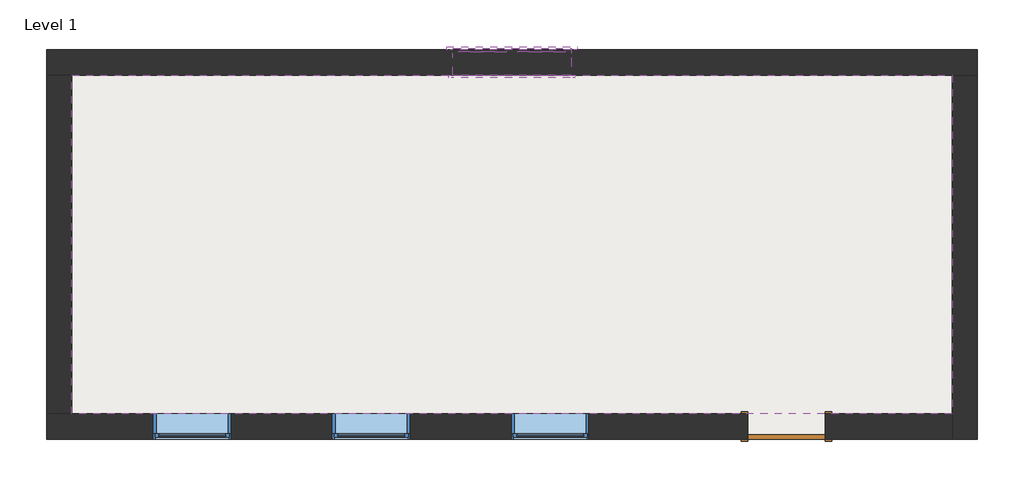
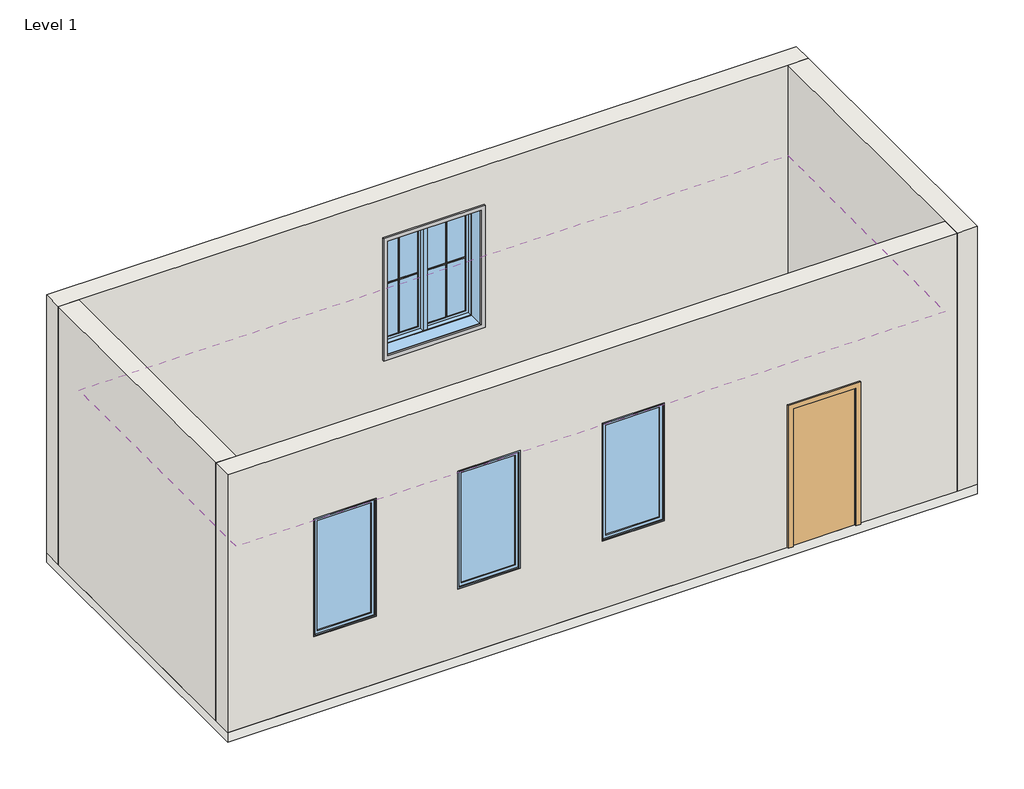
# One storey: 4 proxies, 4 walls, 4 windows, 1 covering, 1 door, 1 slab.
"""IFC4 building model written with IfcOpenShell, lengths in millimetres."""

import ifcopenshell
import ifcopenshell.guid

model = None  # the IFC model being written
_history = None  # IfcOwnerHistory: only IFC2X3 demands one
_inside = {}  # id of a spatial element -> (the spatial element, [elements in it])
_under = {}  # id of a project, library or spatial element -> (it, [spatial elements below it])
_declared = {}  # id of a project -> (the project, [libraries it declares])
_typed = {}  # id of a type object -> (the type object, [elements of that type])
_made_of = {}  # id of a material, layer set ... -> (it, [elements and type objects made of it])


def new_model(schema):
    """Start an empty IFC model of exactly this schema.

    Asked for "IFC4X3", IfcOpenShell would pick the latest addendum, in which some entities
    have other attributes; the version numbers below select the first issue.
    IFC2X3 requires an IfcOwnerHistory on every rooted entity: one is made here for all.
    """
    global model, _history
    if schema == "IFC4X3":
        model = ifcopenshell.file(schema_version=(4, 3, 0, 0))
    else:
        model = ifcopenshell.file(schema=schema)
    _inside.clear()
    _under.clear()
    _declared.clear()
    _typed.clear()
    _made_of.clear()
    _history = None
    if model.schema == "IFC2X3":
        org = make("IfcOrganization", Name="unknown")
        user = make(
            "IfcPersonAndOrganization",
            ThePerson=make("IfcPerson", FamilyName="unknown"),
            TheOrganization=org,
        )
        app = make(
            "IfcApplication",
            ApplicationDeveloper=org,
            Version="unknown",
            ApplicationFullName="unknown",
            ApplicationIdentifier="unknown",
        )
        _history = make(
            "IfcOwnerHistory",
            OwningUser=user,
            OwningApplication=app,
            ChangeAction="ADDED",
            CreationDate=0,
        )
    return model


def make(cls, **values):
    """One entity of the class cls with the attributes given. An attribute that is None is left unset."""
    return model.create_entity(
        cls, **{name: value for name, value in values.items() if value is not None}
    )


def rooted(cls, **values):
    """An entity with a GlobalId (a new one), such as an element, a storey or a relation."""
    return make(cls, GlobalId=ifcopenshell.guid.new(), OwnerHistory=_history, **values)


def si_unit(unit_type, name, prefix=None):
    """IfcSIUnit, for example si_unit("LENGTHUNIT", "METRE", prefix="MILLI")."""
    return make("IfcSIUnit", UnitType=unit_type, Prefix=prefix, Name=name)


def assignment(units):
    """IfcUnitAssignment: the units of a project."""
    return None if units is None else make("IfcUnitAssignment", Units=units)


def point(xyz):
    """IfcCartesianPoint."""
    return None if xyz is None else make("IfcCartesianPoint", Coordinates=xyz)


def direction(xyz):
    """IfcDirection."""
    return None if xyz is None else make("IfcDirection", DirectionRatios=xyz)


def frame(location, z_axis=None, x_axis=None):
    """IfcAxis2Placement3D, a coordinate frame: its origin and axes. An axis left out is left unset."""
    return make(
        "IfcAxis2Placement3D",
        Location=point(location),
        Axis=direction(z_axis),
        RefDirection=direction(x_axis),
    )


def origin():
    """The frame at (0, 0, 0) with its axes left unset."""
    return frame((0.0, 0.0, 0.0))


def origin_with_axes():
    """The frame at (0, 0, 0) with the z axis (0, 0, 1) and the x axis (1, 0, 0) written out."""
    return frame((0.0, 0.0, 0.0), z_axis=(0.0, 0.0, 1.0), x_axis=(1.0, 0.0, 0.0))


def place(relative_to, where):
    """IfcLocalPlacement: puts the frame where relative to a parent placement (None: the world)."""
    return make(
        "IfcLocalPlacement", PlacementRelTo=relative_to, RelativePlacement=where
    )


def context(
    kind, dimensions, precision=None, world=None, true_north=None, identifier=None
):
    """IfcGeometricRepresentationContext, for example the 3D "Model" context."""
    return make(
        "IfcGeometricRepresentationContext",
        ContextIdentifier=identifier,
        ContextType=kind,
        CoordinateSpaceDimension=dimensions,
        Precision=precision,
        WorldCoordinateSystem=world,
        TrueNorth=true_north,
    )


def project(units=None, contexts=None):
    """IfcProject with its units and contexts."""
    return rooted(
        "IfcProject",
        Name="project",
        RepresentationContexts=contexts,
        UnitsInContext=assignment(units),
    )


def spatial(cls, under=None, at=None, **own):
    """A site, building, storey or space (cls), placed at a placement, below another one or the project."""
    s = rooted(cls, ObjectPlacement=at, **own)
    if under is not None:
        _under.setdefault(under.id(), (under, []))[1].append(s)
    return s


def polyline(points):
    """IfcPolyline through the points."""
    return make("IfcPolyline", Points=[point(p) for p in points])


def outline(outer, holes=None, kind="AREA"):
    """IfcArbitraryClosedProfileDef: a profile drawn as a closed curve; with holes, ...WithVoids."""
    if holes is None:
        return make("IfcArbitraryClosedProfileDef", ProfileType=kind, OuterCurve=outer)
    return make(
        "IfcArbitraryProfileDefWithVoids",
        ProfileType=kind,
        OuterCurve=outer,
        InnerCurves=holes,
    )


def extrude(swept, where, along, depth):
    """IfcExtrudedAreaSolid: the profile swept, set in the frame where, extruded along a direction by depth."""
    return make(
        "IfcExtrudedAreaSolid",
        SweptArea=swept,
        Position=where,
        ExtrudedDirection=direction(along),
        Depth=depth,
    )


def faces_of(points, faces, orient=None, outer=None):
    """IfcFace entities. A face is a list of loops; a loop is a list of indices into points, from 0.

    orient and outer hold one flag for each loop. By default every Orientation is true, the
    first loop of a face is its IfcFaceOuterBound and the others are IfcFaceBound.
    """
    made = []
    for i, loops in enumerate(faces):
        bounds = []
        for j, loop in enumerate(loops):
            is_outer = j == 0 if outer is None else outer[i][j]
            bounds.append(
                make(
                    "IfcFaceOuterBound" if is_outer else "IfcFaceBound",
                    Bound=make("IfcPolyLoop", Polygon=[points[k] for k in loop]),
                    Orientation=True if orient is None else orient[i][j],
                )
            )
        made.append(make("IfcFace", Bounds=bounds))
    return made


def faceted_brep(points, faces, orient=None, outer=None, voids=None):
    """IfcFacetedBrep: a solid bounded by flat faces; with voids (closed shells), ...WithVoids."""
    shared = [point(p) for p in points]
    hull = make("IfcClosedShell", CfsFaces=faces_of(shared, faces, orient, outer))
    if voids is None:
        return make("IfcFacetedBrep", Outer=hull)
    return make(
        "IfcFacetedBrepWithVoids",
        Outer=hull,
        Voids=[
            make(cls, CfsFaces=faces_of(shared, fs, o, b)) for cls, fs, o, b in voids
        ],
    )


def shape(context_of_items, identifier, shape_type, items):
    """IfcShapeRepresentation: the items that make up one representation, for example the "Body"."""
    return make(
        "IfcShapeRepresentation",
        ContextOfItems=context_of_items,
        RepresentationIdentifier=identifier,
        RepresentationType=shape_type,
        Items=items,
    )


def source(mapping_origin, context_of_items, identifier, shape_type, items):
    """IfcRepresentationMap: a shape defined once, which mapped items show again and again."""
    return make(
        "IfcRepresentationMap",
        MappingOrigin=mapping_origin,
        MappedRepresentation=shape(context_of_items, identifier, shape_type, items),
    )


def transform(
    local_origin,
    x_axis=None,
    y_axis=None,
    z_axis=None,
    scale=None,
    scale2=None,
    scale3=None,
    uniform=True,
):
    """IfcCartesianTransformationOperator3D, or its non-uniform kind. x_axis, y_axis, z_axis: its Axis1, 2, 3."""
    if uniform:
        return make(
            "IfcCartesianTransformationOperator3D",
            Axis1=direction(x_axis),
            Axis2=direction(y_axis),
            LocalOrigin=point(local_origin),
            Scale=scale,
            Axis3=direction(z_axis),
        )
    return make(
        "IfcCartesianTransformationOperator3DnonUniform",
        Axis1=direction(x_axis),
        Axis2=direction(y_axis),
        LocalOrigin=point(local_origin),
        Scale=scale,
        Axis3=direction(z_axis),
        Scale2=scale2,
        Scale3=scale3,
    )


def mapped(mapping_source, mapping_target):
    """IfcMappedItem: shows the shape of a source again, moved by a transform."""
    return make(
        "IfcMappedItem", MappingSource=mapping_source, MappingTarget=mapping_target
    )


def made_of(thing, what):
    """Note that an element or type object is made of a material, layer set ...; save() writes the relation."""
    if what is not None:
        _made_of.setdefault(what.id(), (what, []))[1].append(thing)
    return thing


def element(
    cls,
    number,
    at=None,
    inside=None,
    cuts=None,
    type_object=None,
    material=None,
    context=None,
    identifier="Body",
    shape_type=None,
    held_by="IfcProductDefinitionShape",
    body=None,
    shapes=None,
    **own,
):
    """One element of the class cls, such as IfcWall. Its Tag is "e" and its number.

    at: its placement. inside: the storey or other place that contains it. cuts: it is an
    opening in that element (IfcRelVoidsElement). A single representation is given by context,
    identifier, shape_type and body (its items); several are given by shapes. held_by: the class
    of the entity that holds the representations. save() writes the other relations.
    """
    e = rooted(cls, Tag="e%d" % number, ObjectPlacement=at, **own)
    if body is not None:
        shapes = [shape(context, identifier, shape_type, body)]
    if shapes is not None:
        e.Representation = make(held_by, Representations=shapes)
    if inside is not None:
        _inside.setdefault(inside.id(), (inside, []))[1].append(e)
    if cuts is not None:
        rooted(
            "IfcRelVoidsElement", RelatingBuildingElement=cuts, RelatedOpeningElement=e
        )
    if type_object is not None:
        _typed.setdefault(type_object.id(), (type_object, []))[1].append(e)
    return made_of(e, material)


def aggregate(whole, parts):
    """IfcRelAggregates: a whole, such as a stair, and the parts it consists of."""
    return rooted("IfcRelAggregates", RelatingObject=whole, RelatedObjects=parts)


def save(model, path):
    """Write the relations noted so far, then the file.

    IfcRelAggregates (storeys below a building ...), IfcRelContainedInSpatialStructure (elements
    in a storey), IfcRelDefinesByType, IfcRelAssociatesMaterial and IfcRelDeclares: one each for
    every whole, place, type object, material and project.
    """
    for whole, parts in _under.values():
        aggregate(whole, parts)
    for where, things in _inside.values():
        rooted(
            "IfcRelContainedInSpatialStructure",
            RelatedElements=things,
            RelatingStructure=where,
        )
    for kind, things in _typed.values():
        rooted("IfcRelDefinesByType", RelatedObjects=things, RelatingType=kind)
    for what, things in _made_of.values():
        rooted("IfcRelAssociatesMaterial", RelatedObjects=things, RelatingMaterial=what)
    for by, libraries in _declared.values():
        rooted("IfcRelDeclares", RelatingContext=by, RelatedDefinitions=libraries)
    model.write(path)


def m_muntin_pattern_2x2_m_muntin_pattern_2x2_d2d4b859(model_context):
    return source(origin(), model_context, "Body", "SweptSolid", [
        extrude(outline(polyline([(836.5, -6.35), (836.5, -281.7375), (823.8, -281.7375), (823.8, -6.35), (0.0, -6.35), (0.0, 6.35), (823.8, 6.35), (823.8, 281.7375), (836.5, 281.7375), (836.5, 6.35), (1660.3, 6.35), (1660.3, -6.35), (836.5, -6.35)])), frame((0.0, 9.525, 0.0), z_axis=(0.0, 1.0, 0.0), x_axis=(0.0, 0.0, 1.0)), (0.0, 0.0, 1.0), 12.7),
        extrude(outline(polyline([(836.5, -6.35), (836.5, -281.7375), (823.8, -281.7375), (823.8, -6.35), (0.0, -6.35), (0.0, 6.35), (823.8, 6.35), (823.8, 281.7375), (836.5, 281.7375), (836.5, 6.35), (1660.3, 6.35), (1660.3, -6.35), (836.5, -6.35)])), frame((0.0, -22.225, 0.0), z_axis=(0.0, 1.0, 0.0), x_axis=(0.0, 0.0, 1.0)), (0.0, 0.0, 1.0), 12.7),
    ])


def m_muntin_pattern_2x2_m_muntin_pattern_2x2_f3921bb5(model_context):
    return source(origin(), model_context, "Body", "SweptSolid", [
        extrude(outline(polyline([(836.5, -6.35), (836.5, -281.7375), (823.8, -281.7375), (823.8, -6.35), (0.0, -6.35), (0.0, 6.35), (823.8, 6.35), (823.8, 281.7375), (836.5, 281.7375), (836.5, 6.35), (1660.3, 6.35), (1660.3, -6.35), (836.5, -6.35)])), frame((0.0, -22.225, 0.0), z_axis=(0.0, 1.0, 0.0), x_axis=(0.0, 0.0, 1.0)), (0.0, 0.0, 1.0), 12.7),
        extrude(outline(polyline([(836.5, -6.35), (836.5, -281.7375), (823.8, -281.7375), (823.8, -6.35), (0.0, -6.35), (0.0, 6.35), (823.8, 6.35), (823.8, 281.7375), (836.5, 281.7375), (836.5, 6.35), (1660.3, 6.35), (1660.3, -6.35), (836.5, -6.35)])), frame((0.0, 9.525, 0.0), z_axis=(0.0, 1.0, 0.0), x_axis=(0.0, 0.0, 1.0)), (0.0, 0.0, 1.0), 12.7),
    ])


def m_trim_window_exterior_flat_with_sill_136e302d(model_context):
    return source(origin(), model_context, "Body", "SweptSolid", [
        extrude(outline(polyline([(760.0, -1820.4323709), (760.0, -1880.4323709), (-760.0, -1880.4323709), (-760.0, -1820.4323709), (760.0, -1820.4323709)])), origin_with_axes(), (0.0, 0.0, 1.0), 19.05),
        extrude(outline(polyline([(-1830.0, 38.1), (-1802.4580645, 38.1), (-1800.0, 19.05), (-1800.0, 0.0), (-1820.4323709, 0.0), (-1820.4323709, 19.05), (-1830.0, 19.05), (-1830.0, 38.1)])), frame((-772.7, 0.0, 0.0), z_axis=(1.0, 0.0, 0.0), x_axis=(0.0, 1.0, 0.0)), (0.0, 0.0, 1.0), 1545.4),
        extrude(outline(polyline([(-760.0, 60.0), (760.0, 60.0), (760.0, -1800.0), (700.0, -1800.0), (700.0, 0.0), (-700.0, 0.0), (-700.0, -1800.0), (-760.0, -1800.0), (-760.0, 60.0)])), origin_with_axes(), (0.0, 0.0, 1.0), 19.05),
    ])


def m_trim_window_interior_flat_picture_frame_c6c50358(model_context):
    return source(origin(), model_context, "Body", "SweptSolid", [
        extrude(outline(polyline([(747.3, 47.3), (747.3, -1847.3), (-747.3, -1847.3), (-747.3, 47.3), (747.3, 47.3)]), holes=[polyline([(687.3, -12.7), (-687.3, -12.7), (-687.3, -1787.3), (687.3, -1787.3), (687.3, -12.7)])]), origin_with_axes(), (0.0, 0.0, 1.0), 30.0),
    ])


def m_single_flush_0915_x_2134mm_9cebaac8(model_context):
    return source(origin(), model_context, "Body", "SweptSolid", [
        extrude(outline(polyline([(2210.0, -533.5), (0.0, -533.5), (0.0, -457.5), (2134.0, -457.5), (2134.0, 457.5), (0.0, 457.5), (0.0, 533.5), (2210.0, 533.5), (2210.0, -533.5)])), frame((0.0, 150.0, 0.0), z_axis=(0.0, 1.0, 0.0), x_axis=(0.0, 0.0, 1.0)), (0.0, 0.0, 1.0), 25.0),
        extrude(outline(polyline([(2210.0, 533.5), (2210.0, -533.5), (0.0, -533.5), (0.0, -457.5), (2134.0, -457.5), (2134.0, 457.5), (0.0, 457.5), (0.0, 533.5), (2210.0, 533.5)])), frame((0.0, -175.0, 0.0), z_axis=(0.0, 1.0, 0.0), x_axis=(0.0, 0.0, 1.0)), (0.0, 0.0, 1.0), 25.0),
        extrude(outline(polyline([(457.5, 99.0), (-457.5, 99.0), (-457.5, 150.0), (457.5, 150.0), (457.5, 99.0)])), origin_with_axes(), (0.0, 0.0, 1.0), 2134.0),
    ])


def m_fixed_0915_x_1830mm_2a137b51(model_context):
    return source(origin(), model_context, "Body", "SweptSolid", [
        extrude(outline(polyline([(-394.5, 128.0), (394.5, 128.0), (394.5, 116.0), (-394.5, 116.0), (-394.5, 128.0)])), frame((0.0, 0.0, 368.0), z_axis=(0.0, 0.0, 1.0), x_axis=(1.0, 0.0, 0.0)), (0.0, 0.0, 1.0), 1704.0),
        extrude(outline(polyline([(2116.0, -438.5), (324.0, -438.5), (324.0, 438.5), (2116.0, 438.5), (2116.0, -438.5)]), holes=[polyline([(2072.0, -394.5), (2072.0, 394.5), (368.0, 394.5), (368.0, -394.5), (2072.0, -394.5)])]), frame((0.0, 100.0, 0.0), z_axis=(0.0, 1.0, 0.0), x_axis=(0.0, 0.0, 1.0)), (0.0, 0.0, 1.0), 44.0),
        extrude(outline(polyline([(2135.0, -457.5), (305.0, -457.5), (305.0, 457.5), (2135.0, 457.5), (2135.0, -457.5)]), holes=[polyline([(2116.0, -438.5), (2116.0, 438.5), (324.0, 438.5), (324.0, -438.5), (2116.0, -438.5)])]), frame((0.0, 100.0, 0.0), z_axis=(0.0, 1.0, 0.0), x_axis=(0.0, 0.0, 1.0)), (0.0, 0.0, 1.0), 63.0),
        extrude(outline(polyline([(2135.0, -457.5), (305.0, -457.5), (305.0, 457.5), (2135.0, 457.5), (2135.0, -457.5)]), holes=[polyline([(2103.0, -425.5), (2103.0, 425.5), (337.0, 425.5), (337.0, -425.5), (2103.0, -425.5)])]), frame((0.0, -137.0, 0.0), z_axis=(0.0, 1.0, 0.0), x_axis=(0.0, 0.0, 1.0)), (0.0, 0.0, 1.0), 237.0),
    ])


def m_window_casement_double_1400_x_1800mm_f8d7c7c6(model_context):
    return source(origin(), model_context, "Body", "SolidModel", [
        faceted_brep([(9.525, 169.05, 2687.3), (-9.525, 169.05, 2687.3), (-9.525, 118.25, 2687.3), (9.525, 118.25, 2687.3), (9.525, 169.05, 912.7), (9.525, 118.25, 912.7), (-9.525, 118.25, 912.7), (-9.525, 169.05, 912.7), (-9.525, 118.25, 931.75), (-9.525, 118.25, 2668.25), (-30.1625, 118.25, 931.75), (-30.1625, 118.25, 2668.25), (-30.1625, 54.75, 931.75), (-30.1625, 54.75, 2668.25), (30.1625, 54.75, 931.75), (30.1625, 54.75, 2668.25), (30.1625, 118.25, 931.75), (30.1625, 118.25, 2668.25), (9.525, 118.25, 931.75), (9.525, 118.25, 2668.25)], [[[0, 1, 2, 3]], [[4, 5, 6, 7]], [[1, 0, 4, 7]], [[2, 1, 7, 6, 8, 9]], [[9, 8, 10, 11]], [[11, 10, 12, 13]], [[13, 12, 14, 15]], [[15, 14, 16, 17]], [[17, 16, 18, 19]], [[0, 3, 19, 18, 5, 4]], [[18, 8, 6, 5]], [[9, 19, 3, 2]], [[8, 18, 16, 14, 12, 10]], [[19, 9, 11, 13, 15, 17]]]),
        extrude(outline(polyline([(-66.675, 150.0), (-66.675, 143.65), (-630.15, 143.65), (-630.15, 150.0), (-66.675, 150.0)])), frame((0.0, 0.0, 969.85), z_axis=(0.0, 0.0, 1.0), x_axis=(1.0, 0.0, 0.0)), (0.0, 0.0, 1.0), 1660.3),
        extrude(outline(polyline([(-630.15, 130.95), (-630.15, 137.3), (-66.675, 137.3), (-66.675, 130.95), (-630.15, 130.95)])), frame((0.0, 0.0, 969.85), z_axis=(0.0, 0.0, 1.0), x_axis=(1.0, 0.0, 0.0)), (0.0, 0.0, 1.0), 1660.3),
        extrude(outline(polyline([(630.15, 150.0), (630.15, 143.65), (66.675, 143.65), (66.675, 150.0), (630.15, 150.0)])), frame((0.0, 0.0, 969.85), z_axis=(0.0, 0.0, 1.0), x_axis=(1.0, 0.0, 0.0)), (0.0, 0.0, 1.0), 1660.3),
        extrude(outline(polyline([(66.675, 130.95), (66.675, 137.3), (630.15, 137.3), (630.15, 130.95), (66.675, 130.95)])), frame((0.0, 0.0, 969.85), z_axis=(0.0, 0.0, 1.0), x_axis=(1.0, 0.0, 0.0)), (0.0, 0.0, 1.0), 1660.3),
        extrude(outline(polyline([(2687.3, -687.3), (912.7, -687.3), (912.7, -9.525), (2687.3, -9.525), (2687.3, -687.3)]), holes=[polyline([(2630.15, -66.675), (969.85, -66.675), (969.85, -630.15), (2630.15, -630.15), (2630.15, -66.675)])]), frame((0.0, 118.25, 0.0), z_axis=(0.0, 1.0, 0.0), x_axis=(0.0, 0.0, 1.0)), (0.0, 0.0, 1.0), 44.45),
        extrude(outline(polyline([(912.7, 687.3), (2687.3, 687.3), (2687.3, 9.525), (912.7, 9.525), (912.7, 687.3)]), holes=[polyline([(969.85, 66.675), (2630.15, 66.675), (2630.15, 630.15), (969.85, 630.15), (969.85, 66.675)])]), frame((0.0, 118.25, 0.0), z_axis=(0.0, 1.0, 0.0), x_axis=(0.0, 0.0, 1.0)), (0.0, 0.0, 1.0), 44.45),
        extrude(outline(polyline([(2700.0, -700.0), (900.0, -700.0), (900.0, 700.0), (2700.0, 700.0), (2700.0, -700.0)]), holes=[polyline([(2680.95, 680.95), (919.05, 680.95), (919.05, -680.95), (2680.95, -680.95), (2680.95, 680.95)])]), frame((0.0, -150.0, 0.0), z_axis=(0.0, 1.0, 0.0), x_axis=(0.0, 0.0, 1.0)), (0.0, 0.0, 1.0), 204.75),
        faceted_brep([(668.25, 118.25, 2668.25), (668.25, 54.75, 2668.25), (-668.25, 54.75, 2668.25), (-668.25, 118.25, 2668.25), (687.3, 169.05, 2687.3), (687.3, 118.25, 2687.3), (-687.3, 118.25, 2687.3), (-687.3, 169.05, 2687.3), (700.0, 54.75, 2700.0), (700.0, 169.05, 2700.0), (-700.0, 169.05, 2700.0), (-700.0, 54.75, 2700.0), (-668.25, 54.75, 931.75), (-668.25, 118.25, 931.75), (-687.3, 118.25, 912.7), (-687.3, 169.05, 912.7), (-700.0, 169.05, 900.0), (-700.0, 54.75, 900.0), (668.25, 54.75, 931.75), (668.25, 118.25, 931.75), (687.3, 118.25, 912.7), (687.3, 169.05, 912.7), (700.0, 169.05, 900.0), (700.0, 54.75, 900.0)], [[[0, 1, 2, 3]], [[4, 5, 6, 7]], [[8, 9, 10, 11]], [[3, 2, 12, 13]], [[7, 6, 14, 15]], [[11, 10, 16, 17]], [[13, 12, 18, 19]], [[15, 14, 20, 21]], [[17, 16, 22, 23]], [[11, 17, 23, 8], [1, 18, 12, 2]], [[19, 18, 1, 0]], [[5, 20, 14, 6], [3, 13, 19, 0]], [[21, 20, 5, 4]], [[23, 22, 9, 8]], [[9, 22, 16, 10], [7, 15, 21, 4]]]),
    ])


model = new_model("IFC4")

# Units and contexts
model_context = context("Model", 3, world=origin())
ifc_project = project(units=[si_unit("LENGTHUNIT", "METRE", prefix="MILLI")], contexts=[model_context])

# Site, building, storey
site = spatial("IfcSite", under=ifc_project)
building = spatial("IfcBuilding", under=site)
storey = spatial("IfcBuildingStorey", under=building, Name="Level 1", Elevation=0.0)

# Proxies
placement = place(None, origin())
m_muntin_pattern_2x2_m_muntin_pattern_2x2_shape = m_muntin_pattern_2x2_m_muntin_pattern_2x2_d2d4b859(model_context)
element("IfcBuildingElementProxy", 1, Name="M_Muntin Pattern_2x2 : M_Muntin Pattern_2x2", ObjectType="M_Muntin Pattern_2x2 : M_Muntin Pattern_2x2", at=placement, inside=storey, context=model_context, shape_type="MappedRepresentation", body=[
    mapped(m_muntin_pattern_2x2_m_muntin_pattern_2x2_shape, transform((3955.3182322, 4425.5280909, 1625.687058), x_axis=(1.0, 0.0, 0.0), y_axis=(0.0, 1.0, 0.0), z_axis=(0.0, 0.0, 1.0))),
])
m_muntin_pattern_2x2_m_muntin_pattern_2x2_2_shape = m_muntin_pattern_2x2_m_muntin_pattern_2x2_f3921bb5(model_context)
element("IfcBuildingElementProxy", 2, Name="M_Muntin Pattern_2x2 : M_Muntin Pattern_2x2", ObjectType="M_Muntin Pattern_2x2 : M_Muntin Pattern_2x2", at=placement, inside=storey, context=model_context, shape_type="MappedRepresentation", body=[
    mapped(m_muntin_pattern_2x2_m_muntin_pattern_2x2_2_shape, transform((4652.1432322, 4425.5280909, 1625.687058), x_axis=(-1.0, 0.0, 0.0), y_axis=(0.0, -1.0, 0.0), z_axis=(0.0, 0.0, 1.0))),
])
m_trim_window_exterior_flat_with_sill_shape = m_trim_window_exterior_flat_with_sill_136e302d(model_context)
element("IfcBuildingElementProxy", 3, Name="M_Trim-Window-Exterior-Flat : with Sill", ObjectType="M_Trim-Window-Exterior-Flat : with Sill", at=placement, inside=storey, context=model_context, shape_type="MappedRepresentation", body=[
    mapped(m_trim_window_exterior_flat_with_sill_shape, transform((4303.7307322, 4435.0530909, 3355.837058), x_axis=(-1.0, 0.0, 0.0), y_axis=(0.0, 0.0, 1.0), z_axis=(0.0, 1.0, 0.0))),
])
m_trim_window_interior_flat_picture_frame_shape = m_trim_window_interior_flat_picture_frame_c6c50358(model_context)
element("IfcBuildingElementProxy", 4, Name="M_Trim-Window-Interior-Flat : Picture Frame", ObjectType="M_Trim-Window-Interior-Flat : Picture Frame", at=placement, inside=storey, context=model_context, shape_type="MappedRepresentation", body=[
    mapped(m_trim_window_interior_flat_picture_frame_shape, transform((4303.7307322, 4135.0530909, 3355.837058), x_axis=(1.0, 0.0, 0.0), y_axis=(0.0, 0.0, 1.0), z_axis=(0.0, -1.0, 0.0))),
])

# Covering
element("IfcCovering", 5, ObjectType="Plain", at=placement, inside=storey, context=model_context, shape_type="SweptSolid", body=[
    extrude(outline(polyline([(-896.2692678, 4135.0530909), (9503.7307322, 4135.0530909), (9503.7307322, 135.0530909), (-896.2692678, 135.0530909), (-896.2692678, 4135.0530909)])), frame((0.0, 0.0, 2600.0), z_axis=(0.0, 0.0, 1.0), x_axis=(1.0, 0.0, 0.0)), (0.0, 0.0, 1.0), 57.0),
])

# Door
m_single_flush_0915_x_2134mm_shape = m_single_flush_0915_x_2134mm_9cebaac8(model_context)
element("IfcDoor", 6, ObjectType="M_Single-Flush : 0915 x 2134mm", at=placement, inside=storey, context=model_context, shape_type="MappedRepresentation", body=[
    mapped(m_single_flush_0915_x_2134mm_shape, transform((7546.2307322, -14.9469091, 0.0), x_axis=(-1.0, 0.0, 0.0), y_axis=(0.0, -1.0, 0.0), z_axis=(0.0, 0.0, 1.0))),
])

# Slab
element("IfcSlab", 7, ObjectType="Generic 150mm", at=placement, inside=storey, context=model_context, shape_type="SweptSolid", body=[
    extrude(outline(polyline([(9803.7307322, 4435.0530909), (9803.7307322, -164.9469091), (-1196.2692678, -164.9469091), (-1196.2692678, 4435.0530909), (9803.7307322, 4435.0530909)])), frame((0.0, 0.0, -150.0), z_axis=(0.0, 0.0, 1.0), x_axis=(1.0, 0.0, 0.0)), (0.0, 0.0, 1.0), 150.0),
])

# Walls
element("IfcWall", 8, ObjectType="Generic - 300mm", at=placement, inside=storey, context=model_context, shape_type="Brep", body=[
    faceted_brep([(-1196.2692678, 4135.0530909, 0.0), (-896.2692678, 4135.0530909, 0.0), (9503.7307322, 4135.0530909, 0.0), (9803.7307322, 4135.0530909, 0.0), (9803.7307322, 4135.0530909, 4000.0), (9503.7307322, 4135.0530909, 4000.0), (-896.2692678, 4135.0530909, 4000.0), (-1196.2692678, 4135.0530909, 4000.0), (5003.7307322, 4135.0530909, 3355.837058), (5003.7307322, 4135.0530909, 1555.837058), (3603.7307322, 4135.0530909, 1555.837058), (3603.7307322, 4135.0530909, 3355.837058), (-1196.2692678, 4435.0530909, 0.0), (-1196.2692678, 4435.0530909, 4000.0), (9803.7307322, 4435.0530909, 4000.0), (9803.7307322, 4435.0530909, 0.0), (5003.7307322, 4435.0530909, 3355.837058), (3603.7307322, 4435.0530909, 3355.837058), (3603.7307322, 4435.0530909, 1555.837058), (5003.7307322, 4435.0530909, 1555.837058)], [[[0, 1, 2, 3, 4, 5, 6, 7], [8, 9, 10, 11]], [[12, 13, 14, 15], [16, 17, 18, 19]], [[3, 2, 1, 0, 12, 15]], [[7, 6, 5, 4, 14, 13]], [[4, 3, 15, 14]], [[0, 7, 13, 12]], [[9, 8, 16, 19]], [[10, 9, 19, 18]], [[11, 10, 18, 17]], [[8, 11, 17, 16]]]),
])
element("IfcWall", 9, ObjectType="Generic - 300mm", at=placement, inside=storey, context=model_context, shape_type="Brep", body=[
    faceted_brep([(9503.7307322, 4135.0530909, 0.0), (9503.7307322, 135.0530909, 0.0), (9503.7307322, -164.9469091, 0.0), (9503.7307322, -164.9469091, 4000.0), (9503.7307322, 135.0530909, 4000.0), (9503.7307322, 4135.0530909, 4000.0), (9803.7307322, 4135.0530909, 0.0), (9803.7307322, 4135.0530909, 4000.0), (9803.7307322, -164.9469091, 4000.0), (9803.7307322, -164.9469091, 0.0)], [[[0, 1, 2, 3, 4, 5]], [[6, 7, 8, 9]], [[2, 1, 0, 6, 9]], [[5, 4, 3, 8, 7]], [[0, 5, 7, 6]], [[3, 2, 9, 8]]]),
])
element("IfcWall", 10, ObjectType="Generic - 300mm", at=placement, inside=storey, context=model_context, shape_type="Brep", body=[
    faceted_brep([(7088.7307322, 135.0530909, 2134.0), (7088.7307322, 135.0530909, 0.0), (-896.2692678, 135.0530909, 0.0), (-1196.2692678, 135.0530909, 0.0), (-1196.2692678, 135.0530909, 4000.0), (-896.2692678, 135.0530909, 4000.0), (9503.7307322, 135.0530909, 4000.0), (9503.7307322, 135.0530909, 0.0), (8003.7307322, 135.0530909, 0.0), (8003.7307322, 135.0530909, 2134.0), (5212.0305123, 135.0530909, 1044.7986801), (5212.0305123, 135.0530909, 2874.7986801), (4297.0305123, 135.0530909, 2874.7986801), (4297.0305123, 135.0530909, 1044.7986801), (3097.0305123, 135.0530909, 1044.7986801), (3097.0305123, 135.0530909, 2874.7986801), (2182.0305123, 135.0530909, 2874.7986801), (2182.0305123, 135.0530909, 1044.7986801), (982.0305123, 135.0530909, 1044.7986801), (982.0305123, 135.0530909, 2874.7986801), (67.0305123, 135.0530909, 2874.7986801), (67.0305123, 135.0530909, 1044.7986801), (-1196.2692678, -164.9469091, 0.0), (7088.7307322, -164.9469091, 0.0), (7088.7307322, -164.9469091, 2134.0), (8003.7307322, -164.9469091, 2134.0), (8003.7307322, -164.9469091, 0.0), (9503.7307322, -164.9469091, 0.0), (9503.7307322, -164.9469091, 4000.0), (-1196.2692678, -164.9469091, 4000.0), (5212.0305123, -164.9469091, 1044.7986801), (4297.0305123, -164.9469091, 1044.7986801), (4297.0305123, -164.9469091, 2874.7986801), (5212.0305123, -164.9469091, 2874.7986801), (3097.0305123, -164.9469091, 1044.7986801), (2182.0305123, -164.9469091, 1044.7986801), (2182.0305123, -164.9469091, 2874.7986801), (3097.0305123, -164.9469091, 2874.7986801), (982.0305123, -164.9469091, 1044.7986801), (67.0305123, -164.9469091, 1044.7986801), (67.0305123, -164.9469091, 2874.7986801), (982.0305123, -164.9469091, 2874.7986801)], [[[0, 1, 2, 3, 4, 5, 6, 7, 8, 9], [10, 11, 12, 13], [14, 15, 16, 17], [18, 19, 20, 21]], [[22, 23, 24, 25, 26, 27, 28, 29], [30, 31, 32, 33], [34, 35, 36, 37], [38, 39, 40, 41]], [[8, 7, 27, 26]], [[3, 2, 1, 23, 22]], [[6, 5, 4, 29, 28]], [[7, 6, 28, 27]], [[4, 3, 22, 29]], [[24, 23, 1, 0]], [[25, 24, 0, 9]], [[26, 25, 9, 8]], [[11, 10, 30, 33]], [[12, 11, 33, 32]], [[13, 12, 32, 31]], [[10, 13, 31, 30]], [[15, 14, 34, 37]], [[16, 15, 37, 36]], [[17, 16, 36, 35]], [[14, 17, 35, 34]], [[19, 18, 38, 41]], [[20, 19, 41, 40]], [[21, 20, 40, 39]], [[18, 21, 39, 38]]]),
])
element("IfcWall", 11, ObjectType="Generic - 300mm", at=placement, inside=storey, context=model_context, shape_type="SweptSolid", body=[
    extrude(outline(polyline([(-896.2692678, 4135.0530909), (-896.2692678, 135.0530909), (-1196.2692678, 135.0530909), (-1196.2692678, 4135.0530909), (-896.2692678, 4135.0530909)])), origin_with_axes(), (0.0, 0.0, 1.0), 4000.0),
])

# Windows
m_fixed_0915_x_1830mm_shape = m_fixed_0915_x_1830mm_2a137b51(model_context)
element("IfcWindow", 12, ObjectType="M_Fixed : 0915 x 1830mm", at=placement, inside=storey, context=model_context, shape_type="MappedRepresentation", body=[
    mapped(m_fixed_0915_x_1830mm_shape, transform((4754.5305123, -1.9469091, 739.7986801), x_axis=(-1.0, 0.0, 0.0), y_axis=(0.0, -1.0, 0.0), z_axis=(0.0, 0.0, 1.0))),
])
element("IfcWindow", 13, ObjectType="M_Fixed : 0915 x 1830mm", at=placement, inside=storey, context=model_context, shape_type="MappedRepresentation", body=[
    mapped(m_fixed_0915_x_1830mm_shape, transform((2639.5305123, -1.9469091, 739.7986801), x_axis=(-1.0, 0.0, 0.0), y_axis=(0.0, -1.0, 0.0), z_axis=(0.0, 0.0, 1.0))),
])
element("IfcWindow", 14, ObjectType="M_Fixed : 0915 x 1830mm", at=placement, inside=storey, context=model_context, shape_type="MappedRepresentation", body=[
    mapped(m_fixed_0915_x_1830mm_shape, transform((524.5305123, -1.9469091, 739.7986801), x_axis=(-1.0, 0.0, 0.0), y_axis=(0.0, -1.0, 0.0), z_axis=(0.0, 0.0, 1.0))),
])
m_window_casement_double_1400_x_1800mm_shape = m_window_casement_double_1400_x_1800mm_f8d7c7c6(model_context)
element("IfcWindow", 15, ObjectType="M_Window-Casement-Double : 1400 x 1800mm", at=placement, inside=storey, context=model_context, shape_type="MappedRepresentation", body=[
    mapped(m_window_casement_double_1400_x_1800mm_shape, transform((4303.7307322, 4285.0530909, 655.837058), x_axis=(1.0, 0.0, 0.0), y_axis=(0.0, 1.0, 0.0), z_axis=(0.0, 0.0, 1.0))),
])

save(model, "model.ifc")

# Revit data of these elements
# Project information
#   Project Issue Date = "Issue Date"
#   Project Status = "Project Status"
#   Client Name = "Owner"
#   Project Address = "Enter address here"
#   Project Name = "Project Name"
#   Project Number = "0001"
# Type "M_Muntin Pattern_2x2 : M_Muntin Pattern_2x2"
#   Width [instance default] = 1200 mm
#   Thickness = 12.7 mm
#   Height [instance default] = 1200 mm
#   Distance = 19.05 mm
#   Interior Material [instance default] = none
#   Exterior Material [instance default] = none
#   Default Elevation = 0
# Type "M_Trim-Window-Exterior-Flat : with Sill"
#   Trim Width = 60 mm
#   Trim Thickness_Picture Frame = 30 mm
#   Trim Thickness_with Sill = 19.05 mm
#   Sill Thickness = 30 mm
#   Opening Width [instance default] = 600 mm
#   Opening Height [instance default] = 900 mm
#   Default Elevation = 1200 mm
#   Sill = yes
#   Picture Frame = no
#   Trim Material [instance default] = none
# Type "M_Trim-Window-Interior-Flat : Picture Frame"
#   Trim Thickness_Picture Frame = 30 mm
#   Trim Width = 60 mm
#   Trim Thickness_with Sill = 20 mm
#   Sill Thickness = 30 mm
#   Opening Width [instance default] = 600 mm
#   Opening Height [instance default] = 900 mm
#   Default Elevation = 1200 mm
#   Sill = no
#   Picture Frame = yes
#   Trim Material [instance default] = none
# Type "Plain"
#   built-in parameter 1002203 = 1 (stored number, unit not read)
#   built-in parameter 1002202 = 1 (stored number, unit not read)
#   Layers, outside or top first: 45 mm "Metal Stud Layer" (function 1); 12 mm "Gypsum Wall Board" (function 1)
# Type "M_Single-Flush : 0915 x 2134mm"
#   Type Mark = "20"
#   Construction Type Id = "MDOOR"
#   Analytic Construction = "Metal"
#   Thickness = 51 mm
#   Thermal Resistance (R) = 0.270117 (m²·K)/W
#   Heat Transfer Coefficient (U) = 3.7021 W/(m²·K)
#   Height = 2134 mm
#   Trim Projection Ext = 25 mm
#   Trim Projection Int = 25 mm
#   Trim Width = 76 mm
#   Width = 915 mm
#   Define Thermal Properties by = 1
#   Define Thermal Properties by = 1
#   Door Material = Door - Panel
#   Frame Material = Door - Frame
#   Visual Light Transmittance = 0
#   Solar Heat Gain Coefficient = 0
#   Function = (empty or 0)
#   Wall Closure = (empty or 0)
# Type "Generic 150mm"
#   Function = 0
#   Layers, outside or top first: 150 mm no material (function 1)
# Type "Generic - 300mm"
#   Layers, outside or top first: 300 mm no material (function 1)
# Type "M_Fixed : 0915 x 1830mm"
#   Type Mark = "18"
#   Construction Type Id = "GSP4R"
#   Analytic Construction = "1/8 in Pilkington single glazing"
#   Visual Light Transmittance = 0.9
#   Thermal Resistance (R) = 0.271106 (m²·K)/W
#   Solar Heat Gain Coefficient = 0.78
#   Heat Transfer Coefficient (U) = 3.6886 W/(m²·K)
#   Height = 1830 mm
#   Default Sill Height = 305 mm
#   Width = 915 mm
#   Window Inset = 19 mm
#   Define Thermal Properties by = 1
#   Define Thermal Properties by = 1
#   Frame Exterior Material = Sash
#   Frame Interior Material = Sash
#   Glass Pane Material = Glass
#   Sash = Sash
#   Wall Closure = (empty or 0)
# Type "M_Window-Casement-Double : 1400 x 1800mm"
#   Type Mark = "26"
#   Fire Rating = "0.5h"
#   Assembly Code = "B2020100"
#   Analytic Construction = "Double glazing - domestic"
#   Frame Extension [instance default] = 6.35 mm
#   Window Inset [instance default] = 0 mm
#   Wall Thickness [instance default] = 150 mm
#   Interior Wall Closure [instance default] = 54.75 mm
#   Half Width = 700 mm
#   Visual Light Transmittance = 0.81
#   Thermal Resistance (R) = 0.319569 (m²·K)/W
#   Solar Heat Gain Coefficient = 0.76
#   Rough Width = 1415 mm
#   Rough Height = 1815 mm
#   Height = 1800 mm
#   Heat Transfer Coefficient (U) = 3.12929 W/(m²·K)
#   Exterior Wall Closure [instance default] = 31.8 mm
#   Extension Jamb [instance default] = 54.75 mm
#   Default Sill Height = 900 mm
#   Width = 1400 mm
#   Define Thermal Properties by = 0
#   Muntin Visibility = yes
#   Interior Trim Visibility [instance default] = yes
#   Exterior Trim Visibility [instance default] = yes
#   Extension Jamb Visibility [instance default] = yes
#   Interior Trim Material = Wood - Stained
#   Muntin Pattern = M_Muntin Pattern_2x2 : M_Muntin Pattern_2x2
#   Interior Trim = M_Trim-Window-Interior-Flat : Picture Frame
#   Interior Frame Material = Wood - Stained
#   Glass Panel Material = Glass
#   Exterior Trim Material = Clad - White
#   Exterior Trim = M_Trim-Window-Exterior-Flat : with Sill
#   Exterior Frame Material = Clad - White
#   Wall Closure = (empty or 0)
# Elements 1, 2 (IfcBuildingElementProxy, "M_Muntin Pattern_2x2 : M_Muntin Pattern_2x2")
#   Width = 563.475 mm
#   Height = 1660.3 mm
#   Interior Material = Wood - Stained
#   Exterior Material = Clad - White
#   Phase Created = New Construction
#   Materials on its faces: "Clad - White", "Wood - Stained"
# Element 3 (IfcBuildingElementProxy, "M_Trim-Window-Exterior-Flat : with Sill")
#   Opening Width = 1400 mm
#   Opening Height = 1800 mm
#   Trim Material = Clad - White
#   Phase Created = New Construction
#   Materials on its faces: "Clad - White"
# Element 4 (IfcBuildingElementProxy, "M_Trim-Window-Interior-Flat : Picture Frame")
#   Opening Width = 1400 mm
#   Opening Height = 1800 mm
#   Trim Material = Wood - Stained
#   Phase Created = New Construction
#   Materials on its faces: "Wood - Stained"
# Element 5 (IfcCovering, "Plain")
#   Height Offset From Level = 2600 mm
#   Phase Created = New Construction
#   Materials on its faces: "Gypsum Wall Board", "Metal Stud Layer"
# Element 6 (IfcDoor, "M_Single-Flush : 0915 x 2134mm")
#   Phase Created = New Construction
#   Materials on its faces: "Door - Frame", "Door - Panel"
# Element 7 (IfcSlab, "Generic 150mm")
#   Height Offset From Level = 0 mm
#   Phase Created = New Construction
#   Materials on its faces: "Default Floor"
# Elements 8, 9, 10, 11 (IfcWall, "Generic - 300mm")
#   Top Offset = 0 mm
#   Base Offset = 0 mm
#   wall height = 4000 mm
#   Phase Created = New Construction
#   Base Constraint = Level 1
#   Top Constraint = Level 2
#   Materials on its faces: "Default Wall"
# Element 12 (IfcWindow, "M_Fixed : 0915 x 1830mm")
#   Mark = "1"
#   Phase Created = New Construction
#   Materials on its faces: "Sash", "Glass"
# Element 13 (IfcWindow, "M_Fixed : 0915 x 1830mm")
#   Mark = "2"
#   Phase Created = New Construction
#   Materials on its faces: "Sash", "Glass"
# Element 14 (IfcWindow, "M_Fixed : 0915 x 1830mm")
#   Mark = "3"
#   Phase Created = New Construction
#   Materials on its faces: "Sash", "Glass"
# Element 15 (IfcWindow, "M_Window-Casement-Double : 1400 x 1800mm")
#   Mark = "4"
#   Window Inset = 0 mm
#   Interior Wall Closure = 54.75 mm
#   Frame Extension = 6.35 mm
#   Exterior Wall Closure = 31.8 mm
#   Interior Trim Visibility = yes
#   Exterior Trim Visibility = yes
#   Phase Created = New Construction
#   Materials on its faces: "Wood - Stained", "Glass", "Clad - White"
# Materials
#   "Metal Stud Layer": class "Metal", colour RGB 127 127 127, transparency 0, Description = "Light gauge steel framing, thermal air layer", Cost = 0
#   "Gypsum Wall Board": class "Generic", colour RGB 249 249 249, transparency 0, Description = "Gypsum Wall Board", Cost = 0
#   "Door - Panel": class "Wood", colour RGB 210 159 95, transparency 0, Cost = 0
#   "Door - Frame": class "Miscellaneous", colour RGB 118 70 51, transparency 0, Cost = 0
#   "Sash": class "Wood", colour RGB 224 178 126, transparency 0, Cost = 0
#   "Glass": class "Glass", colour RGB 0 128 192, transparency 0.9, Description = "Soda Lime Glass", Cost = 0
#   "Wood - Stained": class "Wood", colour RGB 224 178 126, transparency 0, Cost = 0
#   "Clad - White": class "Wood", colour RGB 242 242 238, transparency 0, Cost = 0
#   "Default Floor": class "Miscellaneous", colour RGB 127 127 127, transparency 0, Cost = 0
#   "Default Wall": class "Miscellaneous", colour RGB 128 128 128, transparency 0, Cost = 0
